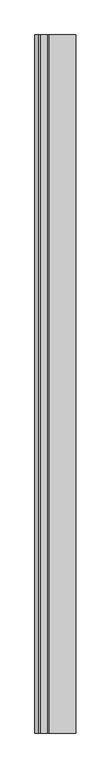
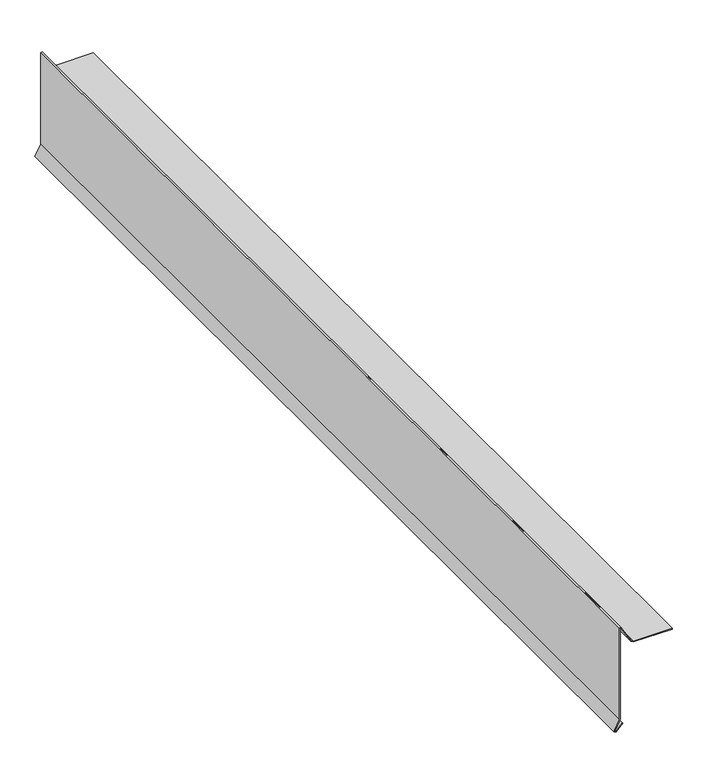
"""IFC4 building model written with IfcOpenShell, lengths in millimetres: proxy geometry, GRAVEL STOP006 14641 : GRAVEL STOP006 14641."""

import ifcopenshell
import ifcopenshell.guid

model = None  # the IFC model being written
_history = None  # IfcOwnerHistory: only IFC2X3 demands one
_inside = {}  # id of a spatial element -> (the spatial element, [elements in it])
_under = {}  # id of a project, library or spatial element -> (it, [spatial elements below it])
_declared = {}  # id of a project -> (the project, [libraries it declares])
_typed = {}  # id of a type object -> (the type object, [elements of that type])
_made_of = {}  # id of a material, layer set ... -> (it, [elements and type objects made of it])


def new_model(schema):
    """Start an empty IFC model of exactly this schema.

    Asked for "IFC4X3", IfcOpenShell would pick the latest addendum, in which some entities
    have other attributes; the version numbers below select the first issue.
    IFC2X3 requires an IfcOwnerHistory on every rooted entity: one is made here for all.
    """
    global model, _history
    if schema == "IFC4X3":
        model = ifcopenshell.file(schema_version=(4, 3, 0, 0))
    else:
        model = ifcopenshell.file(schema=schema)
    _inside.clear()
    _under.clear()
    _declared.clear()
    _typed.clear()
    _made_of.clear()
    _history = None
    if model.schema == "IFC2X3":
        org = make("IfcOrganization", Name="unknown")
        user = make(
            "IfcPersonAndOrganization",
            ThePerson=make("IfcPerson", FamilyName="unknown"),
            TheOrganization=org,
        )
        app = make(
            "IfcApplication",
            ApplicationDeveloper=org,
            Version="unknown",
            ApplicationFullName="unknown",
            ApplicationIdentifier="unknown",
        )
        _history = make(
            "IfcOwnerHistory",
            OwningUser=user,
            OwningApplication=app,
            ChangeAction="ADDED",
            CreationDate=0,
        )
    return model


def make(cls, **values):
    """One entity of the class cls with the attributes given. An attribute that is None is left unset."""
    return model.create_entity(
        cls, **{name: value for name, value in values.items() if value is not None}
    )


def rooted(cls, **values):
    """An entity with a GlobalId (a new one), such as an element, a storey or a relation."""
    return make(cls, GlobalId=ifcopenshell.guid.new(), OwnerHistory=_history, **values)


def si_unit(unit_type, name, prefix=None):
    """IfcSIUnit, for example si_unit("LENGTHUNIT", "METRE", prefix="MILLI")."""
    return make("IfcSIUnit", UnitType=unit_type, Prefix=prefix, Name=name)


def assignment(units):
    """IfcUnitAssignment: the units of a project."""
    return None if units is None else make("IfcUnitAssignment", Units=units)


def point(xyz):
    """IfcCartesianPoint."""
    return None if xyz is None else make("IfcCartesianPoint", Coordinates=xyz)


def direction(xyz):
    """IfcDirection."""
    return None if xyz is None else make("IfcDirection", DirectionRatios=xyz)


def frame(location, z_axis=None, x_axis=None):
    """IfcAxis2Placement3D, a coordinate frame: its origin and axes. An axis left out is left unset."""
    return make(
        "IfcAxis2Placement3D",
        Location=point(location),
        Axis=direction(z_axis),
        RefDirection=direction(x_axis),
    )


def origin():
    """The frame at (0, 0, 0) with its axes left unset."""
    return frame((0.0, 0.0, 0.0))


def place(relative_to, where):
    """IfcLocalPlacement: puts the frame where relative to a parent placement (None: the world)."""
    return make(
        "IfcLocalPlacement", PlacementRelTo=relative_to, RelativePlacement=where
    )


def context(
    kind, dimensions, precision=None, world=None, true_north=None, identifier=None
):
    """IfcGeometricRepresentationContext, for example the 3D "Model" context."""
    return make(
        "IfcGeometricRepresentationContext",
        ContextIdentifier=identifier,
        ContextType=kind,
        CoordinateSpaceDimension=dimensions,
        Precision=precision,
        WorldCoordinateSystem=world,
        TrueNorth=true_north,
    )


def project(units=None, contexts=None):
    """IfcProject with its units and contexts."""
    return rooted(
        "IfcProject",
        Name="project",
        RepresentationContexts=contexts,
        UnitsInContext=assignment(units),
    )


def spatial(cls, under=None, at=None, **own):
    """A site, building, storey or space (cls), placed at a placement, below another one or the project."""
    s = rooted(cls, ObjectPlacement=at, **own)
    if under is not None:
        _under.setdefault(under.id(), (under, []))[1].append(s)
    return s


def polyline(points):
    """IfcPolyline through the points."""
    return make("IfcPolyline", Points=[point(p) for p in points])


def outline(outer, holes=None, kind="AREA"):
    """IfcArbitraryClosedProfileDef: a profile drawn as a closed curve; with holes, ...WithVoids."""
    if holes is None:
        return make("IfcArbitraryClosedProfileDef", ProfileType=kind, OuterCurve=outer)
    return make(
        "IfcArbitraryProfileDefWithVoids",
        ProfileType=kind,
        OuterCurve=outer,
        InnerCurves=holes,
    )


def extrude(swept, where, along, depth):
    """IfcExtrudedAreaSolid: the profile swept, set in the frame where, extruded along a direction by depth."""
    return make(
        "IfcExtrudedAreaSolid",
        SweptArea=swept,
        Position=where,
        ExtrudedDirection=direction(along),
        Depth=depth,
    )


def shape(context_of_items, identifier, shape_type, items):
    """IfcShapeRepresentation: the items that make up one representation, for example the "Body"."""
    return make(
        "IfcShapeRepresentation",
        ContextOfItems=context_of_items,
        RepresentationIdentifier=identifier,
        RepresentationType=shape_type,
        Items=items,
    )


def source(mapping_origin, context_of_items, identifier, shape_type, items):
    """IfcRepresentationMap: a shape defined once, which mapped items show again and again."""
    return make(
        "IfcRepresentationMap",
        MappingOrigin=mapping_origin,
        MappedRepresentation=shape(context_of_items, identifier, shape_type, items),
    )


def transform(
    local_origin,
    x_axis=None,
    y_axis=None,
    z_axis=None,
    scale=None,
    scale2=None,
    scale3=None,
    uniform=True,
):
    """IfcCartesianTransformationOperator3D, or its non-uniform kind. x_axis, y_axis, z_axis: its Axis1, 2, 3."""
    if uniform:
        return make(
            "IfcCartesianTransformationOperator3D",
            Axis1=direction(x_axis),
            Axis2=direction(y_axis),
            LocalOrigin=point(local_origin),
            Scale=scale,
            Axis3=direction(z_axis),
        )
    return make(
        "IfcCartesianTransformationOperator3DnonUniform",
        Axis1=direction(x_axis),
        Axis2=direction(y_axis),
        LocalOrigin=point(local_origin),
        Scale=scale,
        Axis3=direction(z_axis),
        Scale2=scale2,
        Scale3=scale3,
    )


def mapped(mapping_source, mapping_target):
    """IfcMappedItem: shows the shape of a source again, moved by a transform."""
    return make(
        "IfcMappedItem", MappingSource=mapping_source, MappingTarget=mapping_target
    )


def made_of(thing, what):
    """Note that an element or type object is made of a material, layer set ...; save() writes the relation."""
    if what is not None:
        _made_of.setdefault(what.id(), (what, []))[1].append(thing)
    return thing


def element(
    cls,
    number,
    at=None,
    inside=None,
    cuts=None,
    type_object=None,
    material=None,
    context=None,
    identifier="Body",
    shape_type=None,
    held_by="IfcProductDefinitionShape",
    body=None,
    shapes=None,
    **own,
):
    """One element of the class cls, such as IfcWall. Its Tag is "e" and its number.

    at: its placement. inside: the storey or other place that contains it. cuts: it is an
    opening in that element (IfcRelVoidsElement). A single representation is given by context,
    identifier, shape_type and body (its items); several are given by shapes. held_by: the class
    of the entity that holds the representations. save() writes the other relations.
    """
    e = rooted(cls, Tag="e%d" % number, ObjectPlacement=at, **own)
    if body is not None:
        shapes = [shape(context, identifier, shape_type, body)]
    if shapes is not None:
        e.Representation = make(held_by, Representations=shapes)
    if inside is not None:
        _inside.setdefault(inside.id(), (inside, []))[1].append(e)
    if cuts is not None:
        rooted(
            "IfcRelVoidsElement", RelatingBuildingElement=cuts, RelatedOpeningElement=e
        )
    if type_object is not None:
        _typed.setdefault(type_object.id(), (type_object, []))[1].append(e)
    return made_of(e, material)


def aggregate(whole, parts):
    """IfcRelAggregates: a whole, such as a stair, and the parts it consists of."""
    return rooted("IfcRelAggregates", RelatingObject=whole, RelatedObjects=parts)


def save(model, path):
    """Write the relations noted so far, then the file.

    IfcRelAggregates (storeys below a building ...), IfcRelContainedInSpatialStructure (elements
    in a storey), IfcRelDefinesByType, IfcRelAssociatesMaterial and IfcRelDeclares: one each for
    every whole, place, type object, material and project.
    """
    for whole, parts in _under.values():
        aggregate(whole, parts)
    for where, things in _inside.values():
        rooted(
            "IfcRelContainedInSpatialStructure",
            RelatedElements=things,
            RelatingStructure=where,
        )
    for kind, things in _typed.values():
        rooted("IfcRelDefinesByType", RelatedObjects=things, RelatingType=kind)
    for what, things in _made_of.values():
        rooted("IfcRelAssociatesMaterial", RelatedObjects=things, RelatingMaterial=what)
    for by, libraries in _declared.values():
        rooted("IfcRelDeclares", RelatingContext=by, RelatedDefinitions=libraries)
    model.write(path)


def generic_models_072a6e35(model_context):
    return source(origin(), model_context, "Body", "SweptSolid", [
        extrude(outline(polyline([(40077.410403, -2814.9855343), (40091.8049, -2800.5910374), (40092.8027062, -2801.5888435), (40079.2807815, -2815.1107682), (40080.9054201, -2817.2404183), (40101.495749, -2805.9993985), (40293.447969, -2805.9993985), (40293.699878, -2805.0592614), (40258.5078708, -2784.7411466), (40255.9633674, -2780.3339375), (40255.9633674, -2702.4979247), (40257.3744784, -2702.4979247), (40257.3744784, -2779.9558314), (40259.5408757, -2783.7081416), (40295.3431515, -2804.3785952), (40294.5307525, -2807.4105095), (40101.8558531, -2807.4105095), (40080.5182783, -2819.0594785), (40077.410403, -2814.9855343)])), frame((0.0, 999.75, 0.0), z_axis=(0.0, 1.0, 0.0), x_axis=(0.0, 0.0, 1.0)), (0.0, 0.0, 1.0), 2000.25),
    ])


if __name__ == "__main__":
    model = new_model("IFC4")
    model_context = context("Model", 3, world=origin())
    ifc_project = project(units=[si_unit("LENGTHUNIT", "METRE", prefix="MILLI")], contexts=[model_context])
    site = spatial("IfcSite", under=ifc_project)
    building = spatial("IfcBuilding", under=site)
    placement = place(None, origin())
    generic_models_shape = generic_models_072a6e35(model_context)
    element("IfcBuildingElementProxy", 1, Name="GRAVEL STOP006 14641 : GRAVEL STOP006 14641", ObjectType="GRAVEL STOP006 14641 : GRAVEL STOP006 14641", at=placement, inside=building, context=model_context, shape_type="MappedRepresentation", body=[
        mapped(generic_models_shape, transform((0.0, 0.0, 0.0), x_axis=(1.0, 0.0, 0.0), y_axis=(0.0, 1.0, 0.0), z_axis=(0.0, 0.0, 1.0))),
    ])
    save(model, "model.ifc")

# Revit data of these elements
# Type "GRAVEL STOP006 14641 : GRAVEL STOP006 14641"
#   NameOverride = "GRAVEL STOP006"
# Element 1 (IfcBuildingElementProxy, "GRAVEL STOP006 14641 : GRAVEL STOP006 14641")
#   Materials on its faces: "GRAVEL STOP REQUIRED WITH GRAVEL SURFACE SYSTEMS"
# Materials
#   "GRAVEL STOP REQUIRED WITH GRAVEL SURFACE SYSTEMS": class "Unassigned", colour RGB 170 170 127, transparency 0
